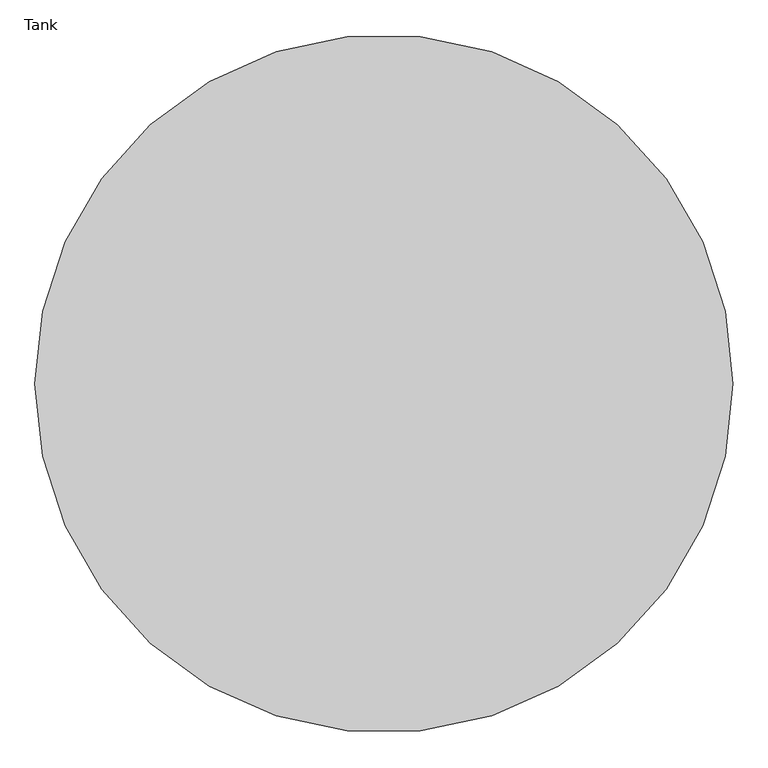
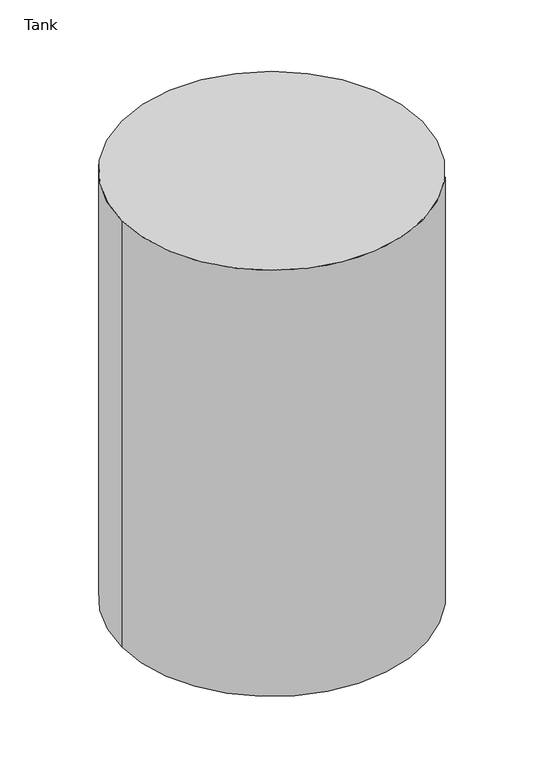
"""IFC4 building model written with IfcOpenShell, lengths in millimetres: proxy geometry, Tank : Future."""

from ifc_helpers import new_model, si_unit, point, origin, origin_with_axes, origin_2d, place, context, project, spatial, circle_curve, trimmed, segment, composite_curve, outline, extrude, source, transform, mapped, element, save


def tank_821d389f(model_context):
    return source(origin(), model_context, "Body", "SweptSolid", [
        extrude(outline(composite_curve([segment(trimmed(circle_curve(origin_2d(), 914.4), [point((-914.4, 0.0))], [point((914.4, 0.0))], False, "CARTESIAN"), True, "CONTINUOUS"), segment(trimmed(circle_curve(origin_2d(), 914.4), [point((914.4, 0.0))], [point((-914.4, 0.0))], False, "CARTESIAN"), True, "CONTINUOUS")], self_intersect=False)), origin_with_axes(), (0.0, 0.0, 1.0), 2743.2),
    ])


if __name__ == "__main__":
    model = new_model("IFC4")
    model_context = context("Model", 3, world=origin())
    ifc_project = project(units=[si_unit("LENGTHUNIT", "METRE", prefix="MILLI")], contexts=[model_context])
    site = spatial("IfcSite", under=ifc_project)
    building = spatial("IfcBuilding", under=site)
    placement = place(None, origin())
    tank_shape = tank_821d389f(model_context)
    element("IfcBuildingElementProxy", 1, Name="Tank : Future", ObjectType="Tank : Future", at=placement, inside=building, context=model_context, shape_type="MappedRepresentation", body=[
        mapped(tank_shape, transform((0.0, 0.0, 0.0), x_axis=(1.0, 0.0, 0.0), y_axis=(0.0, 1.0, 0.0), z_axis=(0.0, 0.0, 1.0))),
    ])
    save(model, "model.ifc")

# Revit data of these elements
# Type "Tank : Future"
#   radius = 3' - 0"
#   Height = 9' - 0"
#   Diameter = 6' - 0"
#   Material = FUTURE
# Element 1 (IfcBuildingElementProxy, "Tank : Future")
#   Materials on its faces: "FUTURE"
# Materials
#   "FUTURE": class "Generic", colour RGB 255 255 255, transparency 0, Cost = 0
